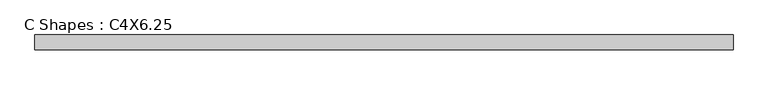
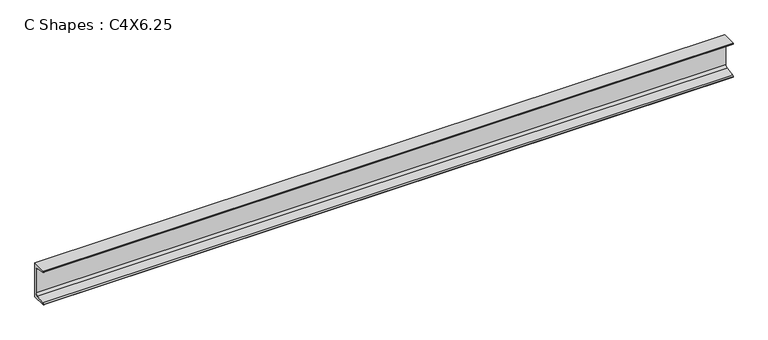
"""IFC4 building model written with IfcOpenShell, lengths in millimetres: beam geometry, C Shapes : C4X6.25."""

from ifc_helpers import new_model, si_unit, point, frame, frame_2d, origin, place, context, project, spatial, polyline, circle_curve, trimmed, segment, composite_curve, outline, extrude, source, transform, mapped, element, save


def c_shapes_c4x6_25_45f65e66(model_context):
    return source(origin(), model_context, "Body", "SweptSolid", [
        extrude(outline(composite_curve([segment(polyline([(11.049, 50.8), (11.049, -50.8), (-30.861, -50.8), (-30.861, -49.7865772)]), True, "CONTINUOUS"), segment(trimmed(circle_curve(frame_2d((-27.4066, -49.7865772)), 3.4544), [point((-30.861, -49.7865772))], [point((-27.9743618, -46.379155))], False, "CARTESIAN"), True, "CONTINUOUS"), segment(polyline([(-27.9743618, -46.379155), (-0.9980765, -41.8842311)]), True, "CONTINUOUS"), segment(trimmed(circle_curve(frame_2d((-2.1336, -35.0693868)), 6.9088), [point((-0.9980765, -41.8842311))], [point((4.7752, -35.0693868))], True, "CARTESIAN"), True, "CONTINUOUS"), segment(polyline([(4.7752, -35.0693868), (4.7752, 35.0693868)]), True, "CONTINUOUS"), segment(trimmed(circle_curve(frame_2d((-2.1336, 35.0693868)), 6.9088), [point((4.7752, 35.0693868))], [point((-0.9980765, 41.8842311))], True, "CARTESIAN"), True, "CONTINUOUS"), segment(polyline([(-0.9980765, 41.8842311), (-27.9743618, 46.379155)]), True, "CONTINUOUS"), segment(trimmed(circle_curve(frame_2d((-27.4066, 49.7865772)), 3.4544), [point((-27.9743618, 46.379155))], [point((-30.861, 49.7865772))], False, "CARTESIAN"), True, "CONTINUOUS"), segment(polyline([(-30.861, 49.7865772), (-30.861, 50.8), (11.049, 50.8)]), True, "CONTINUOUS")], self_intersect=False)), frame((-981.837, 0.0, 0.0), z_axis=(1.0, 0.0, 0.0), x_axis=(0.0, 1.0, 0.0)), (0.0, 0.0, 1.0), 1963.674),
    ])


if __name__ == "__main__":
    model = new_model("IFC4")
    model_context = context("Model", 3, world=origin())
    ifc_project = project(units=[si_unit("LENGTHUNIT", "METRE", prefix="MILLI")], contexts=[model_context])
    site = spatial("IfcSite", under=ifc_project)
    building = spatial("IfcBuilding", under=site)
    placement = place(None, origin())
    c_shapes_c4x6_25_shape = c_shapes_c4x6_25_45f65e66(model_context)
    element("IfcBeam", 1, ObjectType="C Shapes : C4X6.25", at=placement, inside=building, context=model_context, shape_type="MappedRepresentation", body=[
        mapped(c_shapes_c4x6_25_shape, transform((0.0, 0.0, 0.0), x_axis=(1.0, 0.0, 0.0), y_axis=(0.0, 1.0, 0.0), z_axis=(0.0, 0.0, 1.0))),
    ])
    save(model, "model.ifc")

# Revit data of these elements
# Type "C Shapes : C4X6.25"
#   Section Name Key = "ChannelsC4X6.25"
#   Assembly Code = "B10"
#   Width = 1.650"
#   Web Thickness = 0.247"
#   Web Fillet = 0.272"
#   Warping Constant = 1.03 in⁶
#   Torsional Moment of Inertia = 0.0487 in⁴
#   Sloped Flange Angle = 9.46°
#   Section Area = 1.77 in²
#   Plastic Modulus weak axis = 0.569 in³
#   Plastic Modulus strong axis = 2.43 in³
#   Nominal Weight = 6.25 lbf/ft
#   Moment of Inertia weak axis = 0.345 in⁴
#   Moment of Inertia strong axis = 4.00 in⁴
#   Height = 4.000"
#   Flange Thickness Location = 0.7015"
#   Flange Thickness = 0.272"
#   Flange Fillet = 0.136"
#   Elastic Modulus weak axis = 0.284 in³
#   Elastic Modulus strong axis = 2.00 in³
#   Centroid Vertical = 2.000"
#   Centroid Horizontal = 0.435"
#   Length [instance default] = 5' - 0"
#   Structural Material [instance default] = Steel ASTM A36
#   Principal Axes Angle = 0
#   Bolt Spacing = 0
# Element 1 (IfcBeam, "C Shapes : C4X6.25")
#   Materials on its faces: "Steel ASTM A36"
# Materials
#   "Steel ASTM A36": class "Metal", colour RGB 199 199 199, transparency 0, Description = "Structural steel, ASTM A36 Grade B, mill finish", Cost = 0
